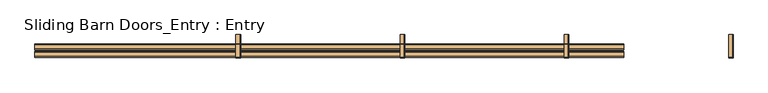
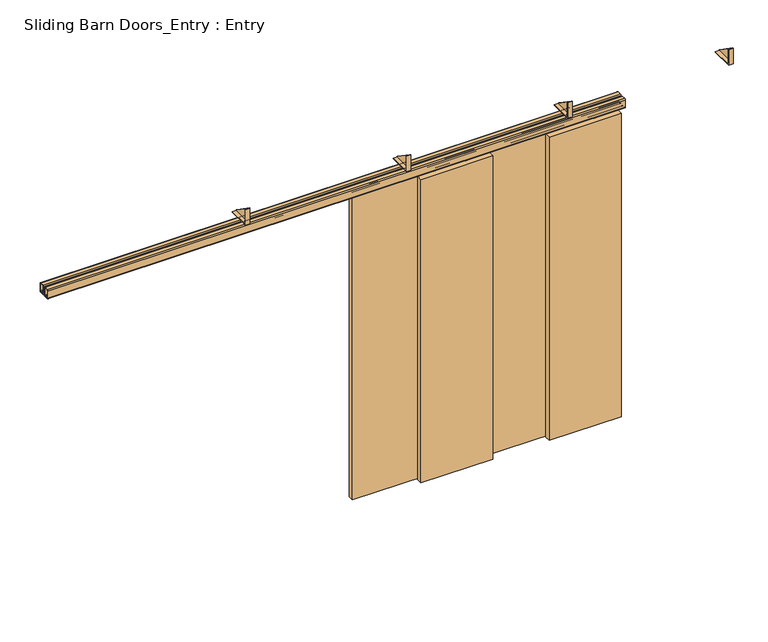
"""IFC4 building model written with IfcOpenShell, lengths in millimetres: door geometry, Sliding Barn Doors_Entry : Entry."""

from ifc_helpers import new_model, si_unit, point, frame, frame_2d, origin, place, context, project, spatial, polyline, circle_curve, trimmed, segment, composite_curve, outline, extrude, source, transform, mapped, element, save


def sliding_barn_doors_entry_entry_3a0c737d(model_context):
    return source(origin(), model_context, "Body", "SweptSolid", [
        extrude(outline(polyline([(222.25, 2149.4037959), (222.25, 2146.3), (79.375, 2146.3), (79.375, 2247.773), (222.25, 2149.4037959)])), frame((521.1795573, 0.0, 0.0), z_axis=(1.0, 0.0, 0.0), x_axis=(0.0, 1.0, 0.0)), (0.0, 0.0, 1.0), 3.175),
        extrude(outline(polyline([(76.2, 2143.125), (76.2, 2247.773), (79.375, 2247.773), (79.375, 2146.3), (222.25, 2146.3), (222.25, 2143.125), (76.2, 2143.125)])), frame((495.878776, 0.0, 0.0), z_axis=(1.0, 0.0, 0.0), x_axis=(0.0, 1.0, 0.0)), (0.0, 0.0, 1.0), 28.4757813),
        extrude(outline(polyline([(222.25, 2149.4037959), (222.25, 2146.3), (79.375, 2146.3), (79.375, 2247.773), (222.25, 2149.4037959)])), frame((-499.053776, 0.0, 0.0), z_axis=(1.0, 0.0, 0.0), x_axis=(0.0, 1.0, 0.0)), (0.0, 0.0, 1.0), 3.175),
        extrude(outline(polyline([(76.2, 2143.125), (76.2, 2247.773), (79.375, 2247.773), (79.375, 2146.3), (222.25, 2146.3), (222.25, 2143.125), (76.2, 2143.125)])), frame((-524.3545573, 0.0, 0.0), z_axis=(1.0, 0.0, 0.0), x_axis=(0.0, 1.0, 0.0)), (0.0, 0.0, 1.0), 28.4757813),
        extrude(outline(polyline([(222.25, 2149.4037959), (222.25, 2146.3), (79.375, 2146.3), (79.375, 2247.773), (222.25, 2149.4037959)])), frame((-1519.2871094, 0.0, 0.0), z_axis=(1.0, 0.0, 0.0), x_axis=(0.0, 1.0, 0.0)), (0.0, 0.0, 1.0), 3.175),
        extrude(outline(polyline([(76.2, 2143.125), (76.2, 2247.773), (79.375, 2247.773), (79.375, 2146.3), (222.25, 2146.3), (222.25, 2143.125), (76.2, 2143.125)])), frame((-1544.5878906, 0.0, 0.0), z_axis=(1.0, 0.0, 0.0), x_axis=(0.0, 1.0, 0.0)), (0.0, 0.0, 1.0), 28.4757812),
        extrude(outline(polyline([(222.25, 2149.4037959), (222.25, 2146.3), (79.375, 2146.3), (79.375, 2247.773), (222.25, 2149.4037959)])), frame((1541.4128906, 0.0, 0.0), z_axis=(1.0, 0.0, 0.0), x_axis=(0.0, 1.0, 0.0)), (0.0, 0.0, 1.0), 3.175),
        extrude(outline(polyline([(76.2, 2143.125), (76.2, 2247.773), (79.375, 2247.773), (79.375, 2146.3), (222.25, 2146.3), (222.25, 2143.125), (76.2, 2143.125)])), frame((1516.1121094, 0.0, 0.0), z_axis=(1.0, 0.0, 0.0), x_axis=(0.0, 1.0, 0.0)), (0.0, 0.0, 1.0), 28.4757812),
        extrude(outline(polyline([(-736.854, 165.1), (-685.546, 165.1), (-685.546, 161.925), (-736.854, 161.925), (-736.854, 165.1)])), frame((0.0, 0.0, 1889.252), z_axis=(0.0, 0.0, 1.0), x_axis=(1.0, 0.0, 0.0)), (0.0, 0.0, 1.0), 168.148),
        extrude(outline(polyline([(-533.654, 165.1), (-482.346, 165.1), (-482.346, 161.925), (-533.654, 161.925), (-533.654, 165.1)])), frame((0.0, 0.0, 1889.252), z_axis=(0.0, 0.0, 1.0), x_axis=(1.0, 0.0, 0.0)), (0.0, 0.0, 1.0), 168.148),
        extrude(outline(polyline([(-330.454, 117.475), (-279.146, 117.475), (-279.146, 114.3), (-330.454, 114.3), (-330.454, 117.475)])), frame((0.0, 0.0, 1889.252), z_axis=(0.0, 0.0, 1.0), x_axis=(1.0, 0.0, 0.0)), (0.0, 0.0, 1.0), 168.148),
        extrude(outline(polyline([(-127.254, 117.475), (-75.946, 117.475), (-75.946, 114.3), (-127.254, 114.3), (-127.254, 117.475)])), frame((0.0, 0.0, 1889.252), z_axis=(0.0, 0.0, 1.0), x_axis=(1.0, 0.0, 0.0)), (0.0, 0.0, 1.0), 168.148),
        extrude(outline(polyline([(126.746, 165.1), (178.054, 165.1), (178.054, 161.925), (126.746, 161.925), (126.746, 165.1)])), frame((0.0, 0.0, 1889.252), z_axis=(0.0, 0.0, 1.0), x_axis=(1.0, 0.0, 0.0)), (0.0, 0.0, 1.0), 168.148),
        extrude(outline(polyline([(279.146, 165.1), (330.454, 165.1), (330.454, 161.925), (279.146, 161.925), (279.146, 165.1)])), frame((0.0, 0.0, 1889.252), z_axis=(0.0, 0.0, 1.0), x_axis=(1.0, 0.0, 0.0)), (0.0, 0.0, 1.0), 168.148),
        extrude(outline(polyline([(482.346, 117.475), (533.654, 117.475), (533.654, 114.3), (482.346, 114.3), (482.346, 117.475)])), frame((0.0, 0.0, 1889.252), z_axis=(0.0, 0.0, 1.0), x_axis=(1.0, 0.0, 0.0)), (0.0, 0.0, 1.0), 168.148),
        extrude(outline(polyline([(685.546, 117.475), (736.854, 117.475), (736.854, 114.3), (685.546, 114.3), (685.546, 117.475)])), frame((0.0, 0.0, 1889.252), z_axis=(0.0, 0.0, 1.0), x_axis=(1.0, 0.0, 0.0)), (0.0, 0.0, 1.0), 168.148),
        extrude(outline(polyline([(-838.2, 161.925), (-381.0, 161.925), (-381.0, 127.0), (-838.2, 127.0), (-838.2, 161.925)])), frame((0.0, 0.0, 25.4), z_axis=(0.0, 0.0, 1.0), x_axis=(1.0, 0.0, 0.0)), (0.0, 0.0, 1.0), 2032.0),
        extrude(outline(polyline([(-25.4, 161.925), (431.8, 161.925), (431.8, 127.0), (-25.4, 127.0), (-25.4, 161.925)])), frame((0.0, 0.0, 25.4), z_axis=(0.0, 0.0, 1.0), x_axis=(1.0, 0.0, 0.0)), (0.0, 0.0, 1.0), 2032.0),
        extrude(outline(polyline([(-431.8, 114.3), (25.4, 114.3), (25.4, 79.375), (-431.8, 79.375), (-431.8, 114.3)])), frame((0.0, 0.0, 25.4), z_axis=(0.0, 0.0, 1.0), x_axis=(1.0, 0.0, 0.0)), (0.0, 0.0, 1.0), 2032.0),
        extrude(outline(polyline([(381.0, 114.3), (838.2, 114.3), (838.2, 79.375), (381.0, 79.375), (381.0, 114.3)])), frame((0.0, 0.0, 25.4), z_axis=(0.0, 0.0, 1.0), x_axis=(1.0, 0.0, 0.0)), (0.0, 0.0, 1.0), 2032.0),
        extrude(outline(composite_curve([segment(polyline([(133.35, 2143.125), (158.877, 2143.125)]), True, "CONTINUOUS"), segment(trimmed(circle_curve(frame_2d((158.877, 2136.775)), 6.35), [point((158.877, 2143.125))], [point((165.227, 2136.775))], False, "CARTESIAN"), True, "CONTINUOUS"), segment(polyline([(165.227, 2136.775), (165.227, 2088.515)]), True, "CONTINUOUS"), segment(trimmed(circle_curve(frame_2d((158.877, 2088.515)), 6.35), [point((165.227, 2088.515))], [point((158.877, 2082.165))], False, "CARTESIAN"), True, "CONTINUOUS"), segment(polyline([(158.877, 2082.165), (153.4683147, 2082.165)]), True, "CONTINUOUS"), segment(trimmed(circle_curve(frame_2d((153.4683147, 2083.7525)), 1.5875), [point((153.4683147, 2082.165))], [point((151.9099816, 2083.4495907))], False, "CARTESIAN"), True, "CONTINUOUS"), segment(polyline([(151.9099816, 2083.4495907), (150.4844659, 2090.7832331), (152.0006029, 2090.7832331), (153.3865251, 2083.6532812), (158.877, 2083.6532812)]), True, "CONTINUOUS"), segment(trimmed(circle_curve(frame_2d((158.877, 2088.515)), 4.8617187), [point((158.877, 2083.6532812))], [point((163.7387188, 2088.515))], True, "CARTESIAN"), True, "CONTINUOUS"), segment(polyline([(163.7387188, 2088.515), (163.7387188, 2136.775)]), True, "CONTINUOUS"), segment(trimmed(circle_curve(frame_2d((158.877, 2136.775)), 4.8617188), [point((163.7387188, 2136.775))], [point((158.877, 2141.6367187))], True, "CARTESIAN"), True, "CONTINUOUS"), segment(polyline([(158.877, 2141.6367187), (133.35, 2141.6367187)]), True, "CONTINUOUS"), segment(trimmed(circle_curve(frame_2d((133.35, 2136.775)), 4.8617187), [point((133.35, 2141.6367187))], [point((128.4882813, 2136.775))], True, "CARTESIAN"), True, "CONTINUOUS"), segment(polyline([(128.4882813, 2136.775), (128.4882813, 2088.515)]), True, "CONTINUOUS"), segment(trimmed(circle_curve(frame_2d((133.35, 2088.515)), 4.8617187), [point((128.4882813, 2088.515))], [point((133.35, 2083.6532812))], True, "CARTESIAN"), True, "CONTINUOUS"), segment(polyline([(133.35, 2083.6532812), (138.8404749, 2083.6532812), (140.2263971, 2090.7832331), (141.7425341, 2090.7832331), (140.3170184, 2083.4495907)]), True, "CONTINUOUS"), segment(trimmed(circle_curve(frame_2d((138.7586853, 2083.7525)), 1.5875), [point((140.3170184, 2083.4495907))], [point((138.7586853, 2082.165))], False, "CARTESIAN"), True, "CONTINUOUS"), segment(polyline([(138.7586853, 2082.165), (133.35, 2082.165)]), True, "CONTINUOUS"), segment(trimmed(circle_curve(frame_2d((133.35, 2088.515)), 6.35), [point((133.35, 2082.165))], [point((127.0, 2088.515))], False, "CARTESIAN"), True, "CONTINUOUS"), segment(polyline([(127.0, 2088.515), (127.0, 2136.775)]), True, "CONTINUOUS"), segment(trimmed(circle_curve(frame_2d((133.35, 2136.775)), 6.35), [point((127.0, 2136.775))], [point((133.35, 2143.125))], False, "CARTESIAN"), True, "CONTINUOUS")], self_intersect=False)), frame((-2794.0, 0.0, 0.0), z_axis=(1.0, 0.0, 0.0), x_axis=(0.0, 1.0, 0.0)), (0.0, 0.0, 1.0), 3657.6),
        extrude(outline(composite_curve([segment(polyline([(85.725, 2143.125), (111.252, 2143.125)]), True, "CONTINUOUS"), segment(trimmed(circle_curve(frame_2d((111.252, 2136.775)), 6.35), [point((111.252, 2143.125))], [point((117.602, 2136.775))], False, "CARTESIAN"), True, "CONTINUOUS"), segment(polyline([(117.602, 2136.775), (117.602, 2088.515)]), True, "CONTINUOUS"), segment(trimmed(circle_curve(frame_2d((111.252, 2088.515)), 6.35), [point((117.602, 2088.515))], [point((111.252, 2082.165))], False, "CARTESIAN"), True, "CONTINUOUS"), segment(polyline([(111.252, 2082.165), (105.8433147, 2082.165)]), True, "CONTINUOUS"), segment(trimmed(circle_curve(frame_2d((105.8433147, 2083.7525)), 1.5875), [point((105.8433147, 2082.165))], [point((104.2849816, 2083.4495907))], False, "CARTESIAN"), True, "CONTINUOUS"), segment(polyline([(104.2849816, 2083.4495907), (102.8594659, 2090.7832331), (104.3756029, 2090.7832331), (105.7615251, 2083.6532812), (111.252, 2083.6532812)]), True, "CONTINUOUS"), segment(trimmed(circle_curve(frame_2d((111.252, 2088.515)), 4.8617187), [point((111.252, 2083.6532812))], [point((116.1137188, 2088.515))], True, "CARTESIAN"), True, "CONTINUOUS"), segment(polyline([(116.1137188, 2088.515), (116.1137188, 2136.775)]), True, "CONTINUOUS"), segment(trimmed(circle_curve(frame_2d((111.252, 2136.775)), 4.8617187), [point((116.1137188, 2136.775))], [point((111.252, 2141.6367187))], True, "CARTESIAN"), True, "CONTINUOUS"), segment(polyline([(111.252, 2141.6367187), (85.725, 2141.6367187)]), True, "CONTINUOUS"), segment(trimmed(circle_curve(frame_2d((85.725, 2136.775)), 4.8617187), [point((85.725, 2141.6367187))], [point((80.8632813, 2136.775))], True, "CARTESIAN"), True, "CONTINUOUS"), segment(polyline([(80.8632813, 2136.775), (80.8632813, 2088.515)]), True, "CONTINUOUS"), segment(trimmed(circle_curve(frame_2d((85.725, 2088.515)), 4.8617187), [point((80.8632813, 2088.515))], [point((85.725, 2083.6532812))], True, "CARTESIAN"), True, "CONTINUOUS"), segment(polyline([(85.725, 2083.6532812), (91.2154749, 2083.6532812), (92.6013971, 2090.7832331), (94.1175341, 2090.7832331), (92.6920184, 2083.4495907)]), True, "CONTINUOUS"), segment(trimmed(circle_curve(frame_2d((91.1336853, 2083.7525)), 1.5875), [point((92.6920184, 2083.4495907))], [point((91.1336853, 2082.165))], False, "CARTESIAN"), True, "CONTINUOUS"), segment(polyline([(91.1336853, 2082.165), (85.725, 2082.165)]), True, "CONTINUOUS"), segment(trimmed(circle_curve(frame_2d((85.725, 2088.515)), 6.35), [point((85.725, 2082.165))], [point((79.375, 2088.515))], False, "CARTESIAN"), True, "CONTINUOUS"), segment(polyline([(79.375, 2088.515), (79.375, 2136.775)]), True, "CONTINUOUS"), segment(trimmed(circle_curve(frame_2d((85.725, 2136.775)), 6.35), [point((79.375, 2136.775))], [point((85.725, 2143.125))], False, "CARTESIAN"), True, "CONTINUOUS")], self_intersect=False)), frame((-2794.0, 0.0, 0.0), z_axis=(1.0, 0.0, 0.0), x_axis=(0.0, 1.0, 0.0)), (0.0, 0.0, 1.0), 3657.6),
    ])


if __name__ == "__main__":
    model = new_model("IFC4")
    model_context = context("Model", 3, world=origin())
    ifc_project = project(units=[si_unit("LENGTHUNIT", "METRE", prefix="MILLI")], contexts=[model_context])
    site = spatial("IfcSite", under=ifc_project)
    building = spatial("IfcBuilding", under=site)
    placement = place(None, origin())
    sliding_barn_doors_entry_entry_shape = sliding_barn_doors_entry_entry_3a0c737d(model_context)
    element("IfcDoor", 1, ObjectType="Sliding Barn Doors_Entry : Entry", at=placement, inside=building, context=model_context, shape_type="MappedRepresentation", body=[
        mapped(sliding_barn_doors_entry_entry_shape, transform((0.0, 0.0, 0.0), x_axis=(1.0, 0.0, 0.0), y_axis=(0.0, 1.0, 0.0), z_axis=(0.0, 0.0, 1.0))),
    ])
    save(model, "model.ifc")

# Revit data of these elements
# Type "Sliding Barn Doors_Entry : Entry"
#   Type Mark = "48"
#   OD_DS_Door_Type = "SLIDER"
#   Analytic Construction = "<None>"
#   rail_overlap_left = 0' - 1"
#   rail_length = 12' - 0"
#   overlap_left = 0' - 0"
#   overlap = 0' - 2"
#   bracket_right = 0' - 9"
#   bracket_left = 0' - 4"
#   Thickness = 0' - 1 3/8"
#   Panel Width = 1' - 6"
#   Panel Height = 6' - 8"
#   Gap 2 = 0' - 0 1/2"
#   Gap 1 = 0' - 0 7/8"
#   Frame Projection Ext. = 0' - 1"
#   Frame Projection Int. = 0' - 1"
#   Frame Width = 0' - 3"
#   Height = 6' - 5 3/8"
#   Width = 5' - 6"
#   Bracket_offset = 0' - 5"
#   Door_4 = yes
#   Door_3 = yes
#   Hardware Material = Metal - Aluminum
#   Door Material = Closet_1
#   Function = (empty or 0)
#   Wall Closure = (empty or 0)
# Element 1 (IfcDoor, "Sliding Barn Doors_Entry : Entry")
#   Materials on its faces: "Metal - Aluminum", "Closet_1"
# Materials
#   "Metal - Aluminum": class "Metal", colour RGB 247 247 247, transparency 0
#   "Closet_1": class "Paint", colour RGB 200 194 183, transparency 0, Cost = 0
